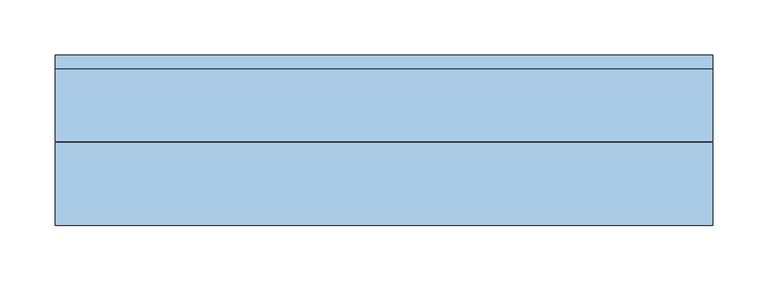
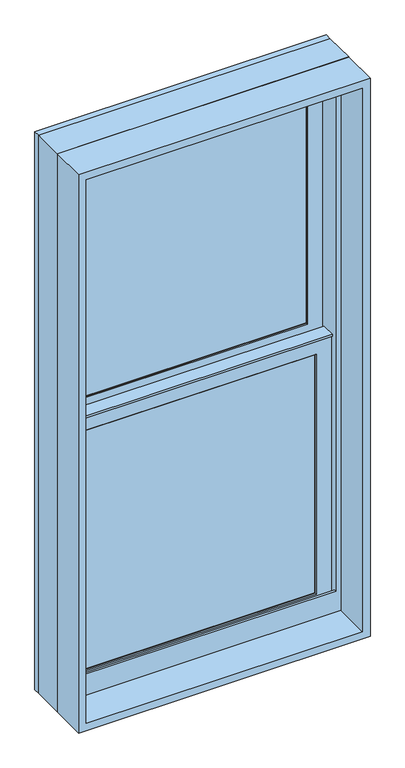
"""IFC4 building model written with IfcOpenShell, lengths in millimetres: window geometry, Window-Double_Hung-Marvin-Essential : ESDH2040."""

from ifc_helpers import new_model, si_unit, frame, origin, place, context, project, spatial, polyline, outline, extrude, faceted_brep, source, transform, mapped, element, save


def window_2436dc5c(model_context):
    return source(origin(), model_context, "Body", "SolidModel", [
        extrude(outline(polyline([(89.9583333, 20.6375), (89.9583333, 15.875), (70.9083333, 15.875), (70.9083333, 20.6375), (89.9583333, 20.6375)])), frame((0.0, 0.0, 1289.05), z_axis=(0.0, 0.0, 1.0), x_axis=(1.0, 0.0, 0.0)), (0.0, 0.0, 1.0), 527.05),
        extrude(outline(polyline([(-70.9083333, 20.6375), (-70.9083333, 15.875), (-89.9583333, 15.875), (-89.9583333, 20.6375), (-70.9083333, 20.6375)])), frame((0.0, 0.0, 1289.05), z_axis=(0.0, 0.0, 1.0), x_axis=(1.0, 0.0, 0.0)), (0.0, 0.0, 1.0), 527.05),
        extrude(outline(polyline([(241.3, 20.6375), (241.3, 15.875), (-241.3, 15.875), (-241.3, 20.6375), (241.3, 20.6375)])), frame((0.0, 0.0, 1543.05), z_axis=(0.0, 0.0, 1.0), x_axis=(1.0, 0.0, 0.0)), (0.0, 0.0, 1.0), 19.05),
        extrude(outline(polyline([(-89.9583333, 46.83125), (-89.9583333, 51.59375), (-70.9083333, 51.59375), (-70.9083333, 46.83125), (-89.9583333, 46.83125)])), frame((0.0, 0.0, 1854.2), z_axis=(0.0, 0.0, 1.0), x_axis=(1.0, 0.0, 0.0)), (0.0, 0.0, 1.0), 527.05),
        extrude(outline(polyline([(70.9083333, 46.83125), (70.9083333, 51.59375), (89.9583333, 51.59375), (89.9583333, 46.83125), (70.9083333, 46.83125)])), frame((0.0, 0.0, 1854.2), z_axis=(0.0, 0.0, 1.0), x_axis=(1.0, 0.0, 0.0)), (0.0, 0.0, 1.0), 527.05),
        extrude(outline(polyline([(-241.3, 46.83125), (-241.3, 51.59375), (241.3, 51.59375), (241.3, 46.83125), (-241.3, 46.83125)])), frame((0.0, 0.0, 2108.2), z_axis=(0.0, 0.0, 1.0), x_axis=(1.0, 0.0, 0.0)), (0.0, 0.0, 1.0), 19.05),
        extrude(outline(polyline([(89.9583333, 20.6375), (70.9083333, 20.6375), (70.9083333, 25.4), (89.9583333, 25.4), (89.9583333, 20.6375)])), frame((0.0, 0.0, 1289.05), z_axis=(0.0, 0.0, 1.0), x_axis=(1.0, 0.0, 0.0)), (0.0, 0.0, 1.0), 527.05),
        extrude(outline(polyline([(-70.9083333, 20.6375), (-89.9583333, 20.6375), (-89.9583333, 25.4), (-70.9083333, 25.4), (-70.9083333, 20.6375)])), frame((0.0, 0.0, 1289.05), z_axis=(0.0, 0.0, 1.0), x_axis=(1.0, 0.0, 0.0)), (0.0, 0.0, 1.0), 527.05),
        extrude(outline(polyline([(241.3, 20.6375), (-241.3, 20.6375), (-241.3, 25.4), (241.3, 25.4), (241.3, 20.6375)])), frame((0.0, 0.0, 1543.05), z_axis=(0.0, 0.0, 1.0), x_axis=(1.0, 0.0, 0.0)), (0.0, 0.0, 1.0), 19.05),
        extrude(outline(polyline([(-89.9583333, 56.35625), (-70.9083333, 56.35625), (-70.9083333, 51.59375), (-89.9583333, 51.59375), (-89.9583333, 56.35625)])), frame((0.0, 0.0, 1854.2), z_axis=(0.0, 0.0, 1.0), x_axis=(1.0, 0.0, 0.0)), (0.0, 0.0, 1.0), 527.05),
        extrude(outline(polyline([(70.9083333, 56.35625), (89.9583333, 56.35625), (89.9583333, 51.59375), (70.9083333, 51.59375), (70.9083333, 56.35625)])), frame((0.0, 0.0, 1854.2), z_axis=(0.0, 0.0, 1.0), x_axis=(1.0, 0.0, 0.0)), (0.0, 0.0, 1.0), 527.05),
        extrude(outline(polyline([(-241.3, 56.35625), (241.3, 56.35625), (241.3, 51.59375), (-241.3, 51.59375), (-241.3, 56.35625)])), frame((0.0, 0.0, 2108.2), z_axis=(0.0, 0.0, 1.0), x_axis=(1.0, 0.0, 0.0)), (0.0, 0.0, 1.0), 19.05),
        faceted_brep([(-268.2875, 5.6780605, 1846.1351748), (-268.2875, 5.6780605, 1841.5), (268.2875, 5.6780605, 1841.5), (268.2875, 5.6780605, 1846.1351748), (-268.2875, 34.8118605, 1846.1351748), (268.2875, 34.8118605, 1846.1351748), (268.2875, 34.8118605, 1841.5), (-268.2875, 34.8118605, 1841.5), (-268.2875, 30.1625, 1841.5), (-268.2875, 30.1625, 1262.0625), (-268.2875, 8.9241104, 1262.0625), (-268.2875, 8.9241104, 1841.5), (268.2875, 8.9241104, 1841.5), (268.2875, 30.1625, 1841.5), (268.2875, 8.9241104, 1262.0625), (268.2875, 30.1625, 1262.0625), (-252.4034752, 11.90625, 1827.2034752), (-252.4034752, 30.1625, 1827.2034752), (252.4034752, 30.1625, 1827.2034752), (252.4034752, 11.90625, 1827.2034752), (-235.74375, 10.4662439, 1810.54375), (-235.74375, 11.90625, 1810.54375), (235.74375, 11.90625, 1810.54375), (235.74375, 10.4662439, 1810.54375), (237.2858834, 8.9241104, 1812.0858834), (-237.2858834, 8.9241104, 1812.0858834), (252.4034752, 30.1625, 1277.9465248), (252.4034752, 11.90625, 1277.9465248), (235.74375, 11.90625, 1294.60625), (235.74375, 10.4662439, 1294.60625), (237.2858834, 8.9241104, 1293.0641166), (-252.4034752, 30.1625, 1277.9465248), (-252.4034752, 11.90625, 1277.9465248), (-235.74375, 11.90625, 1294.60625), (-235.74375, 10.4662439, 1294.60625), (-237.2858834, 8.9241104, 1293.0641166)], [[[0, 1, 2, 3]], [[4, 5, 6, 7]], [[1, 0, 4, 7, 8, 9, 10, 11]], [[2, 1, 11, 12]], [[7, 6, 13, 8]], [[3, 2, 12, 14, 15, 13, 6, 5]], [[0, 3, 5, 4]], [[16, 17, 18, 19]], [[20, 21, 22, 23]], [[20, 23, 24, 25]], [[19, 18, 26, 27]], [[23, 22, 28, 29]], [[24, 23, 29, 30]], [[27, 26, 31, 32]], [[29, 28, 33, 34]], [[30, 29, 34, 35]], [[15, 14, 10, 9]], [[15, 9, 8, 13], [18, 17, 31, 26]], [[17, 16, 32, 31]], [[16, 19, 27, 32], [22, 21, 33, 28]], [[21, 20, 34, 33]], [[20, 25, 35, 34]], [[10, 14, 12, 11], [25, 24, 30, 35]]]),
        extrude(outline(polyline([(38.5955581, 1827.2125), (33.5778968, 1827.2125), (33.5778968, 1828.8), (39.9405976, 1828.8), (39.9405976, 1827.2125), (61.515625, 1827.2125), (47.6307501, 1823.8975159), (38.5955581, 1823.8975159), (38.5955581, 1827.2125)])), frame((-268.2875, 0.0, 0.0), z_axis=(1.0, 0.0, 0.0), x_axis=(0.0, 1.0, 0.0)), (0.0, 0.0, 1.0), 536.575),
        faceted_brep([(298.45, 0.0, 1231.9), (298.45, 0.0, 2438.4), (-298.45, 0.0, 2438.4), (-298.45, 0.0, 1231.9), (272.25625, 0.0, 1293.01875), (-272.25625, 0.0, 1293.01875), (-272.25625, 0.0, 2412.20625), (272.25625, 0.0, 2412.20625), (272.25625, 3.96875, 1231.9), (-272.25625, 3.96875, 1231.9), (-272.25625, 3.96875, 1293.01875), (272.25625, 3.96875, 1293.01875), (-298.45, 65.6828125, 1231.9), (-272.25625, 65.6828125, 1231.9), (272.25625, 65.6828125, 1231.9), (298.45, 65.6828125, 1231.9), (-298.45, 65.6828125, 2438.4), (298.45, 65.6828125, 2438.4), (272.25625, 65.6828125, 2412.20625), (-272.25625, 65.6828125, 2412.20625)], [[[0, 1, 2, 3], [4, 5, 6, 7]], [[8, 9, 10, 11]], [[5, 4, 11, 10]], [[0, 3, 12, 13, 9, 8, 14, 15]], [[13, 12, 16, 17, 15, 14, 18, 19]], [[13, 19, 6, 5, 10, 9]], [[7, 6, 19, 18]], [[18, 14, 8, 11, 4, 7]], [[1, 0, 15, 17]], [[2, 1, 17, 16]], [[3, 2, 16, 12]]]),
        faceted_brep([(272.25625, 30.1625, 1835.15), (270.66875, 30.1625, 1835.15), (270.66875, 30.1625, 1256.2544613), (272.25625, 30.1625, 1256.2544613), (-270.66875, 30.1625, 1835.15), (-272.25625, 30.1625, 1835.15), (-272.25625, 30.1625, 1256.2544613), (-270.66875, 30.1625, 1256.2544613), (270.66875, 63.5, 1835.15), (272.25625, 63.5, 1835.15), (272.25625, 63.5, 1249.7743077), (270.66875, 63.5, 1249.7743077), (-272.25625, 63.5, 1835.15), (-270.66875, 63.5, 1835.15), (-270.66875, 63.5, 1249.7743077), (-272.25625, 63.5, 1249.7743077), (283.5108932, 3.96875, 1261.3460105), (283.5108932, 3.96875, 1231.9), (283.5108932, 65.6828125, 1231.9), (283.5108932, 65.6828125, 1249.350012), (-283.5108932, 3.96875, 1231.9), (-283.5108932, 3.96875, 1261.3460105), (-283.5108932, 65.6828125, 1249.350012), (-283.5108932, 65.6828125, 1231.9), (283.5108932, 78.58125, 1246.8428097), (-283.5108932, 78.58125, 1246.8428097), (-281.4971252, 68.2348864, 1248.8539391), (-263.53135, 68.2348864, 1248.8539391), (-263.53135, 65.6828125, 1249.350012), (263.53135, 65.6828125, 1249.350012), (263.53135, 68.2348864, 1248.8539391), (281.4971252, 68.2348864, 1248.8539391), (-298.45, 65.6828125, 1231.9), (-298.45, 78.5948249, 1231.9), (298.45, 78.5948249, 1231.9), (298.45, 65.6828125, 1231.9), (-298.45, 78.58125, 2438.4), (298.45, 78.58125, 2438.4), (283.5108932, 78.58125, 2423.4608932), (-283.5108932, 78.58125, 2423.4608932), (-298.45, 65.6828125, 2438.4), (-281.4971252, 68.2348864, 2421.4471252), (281.4971252, 68.2348864, 2421.4471252), (263.53135, 68.2348864, 2403.48135), (-263.53135, 68.2348864, 2403.48135), (-263.53135, 65.6828125, 2403.48135), (263.53135, 65.6828125, 2403.48135), (298.45, 65.6828125, 2438.4)], [[[0, 1, 2, 3]], [[4, 5, 6, 7]], [[8, 9, 10, 11]], [[12, 13, 14, 15]], [[1, 8, 11, 2]], [[9, 0, 3, 10]], [[1, 0, 9, 8]], [[5, 4, 13, 12]], [[5, 12, 15, 6]], [[13, 4, 7, 14]], [[16, 17, 18, 19]], [[20, 21, 22, 23]], [[24, 25, 26, 27, 28, 22, 21, 16, 19, 29, 30, 31], [3, 2, 11, 10], [7, 6, 15, 14]], [[17, 16, 21, 20]], [[17, 20, 23, 32, 33, 34, 35, 18]], [[34, 33, 36, 37], [25, 24, 38, 39]], [[33, 32, 40, 36]], [[39, 41, 26, 25]], [[41, 42, 31, 30, 43, 44, 27, 26]], [[44, 45, 28, 27]], [[40, 32, 23, 22, 28, 45, 46, 29, 19, 18, 35, 47]], [[36, 40, 47, 37]], [[39, 38, 42, 41]], [[44, 43, 46, 45]], [[34, 37, 47, 35]], [[42, 38, 24, 31]], [[46, 43, 30, 29]]]),
        extrude(outline(polyline([(248.44375, 11.90625), (-248.44375, 11.90625), (-248.44375, 15.08125), (248.44375, 15.08125), (248.44375, 11.90625)])), frame((0.0, 0.0, 1281.90625), z_axis=(0.0, 0.0, 1.0), x_axis=(1.0, 0.0, 0.0)), (0.0, 0.0, 1.0), 541.3375),
        extrude(outline(polyline([(248.44375, 42.8625), (-248.44375, 42.8625), (-248.44375, 46.0375), (248.44375, 46.0375), (248.44375, 42.8625)])), frame((0.0, 0.0, 1847.05625), z_axis=(0.0, 0.0, 1.0), x_axis=(1.0, 0.0, 0.0)), (0.0, 0.0, 1.0), 541.3375),
        faceted_brep([(-235.74375, 31.194477, 1810.54375), (-237.2858834, 32.7366104, 1812.0858834), (237.2858834, 32.7366104, 1812.0858834), (235.74375, 31.194477, 1810.54375), (-235.74375, 30.1625, 1810.54375), (235.74375, 30.1625, 1810.54375), (-268.2875, 32.7366104, 1843.0875), (-268.2875, 30.1625, 1843.0875), (268.2875, 30.1625, 1843.0875), (268.2875, 32.7366104, 1843.0875), (237.2858834, 32.7366104, 1293.0641166), (235.74375, 31.194477, 1294.60625), (235.74375, 30.1625, 1294.60625), (268.2875, 30.1625, 1262.0625), (268.2875, 32.7366104, 1262.0625), (-237.2858834, 32.7366104, 1293.0641166), (-235.74375, 31.194477, 1294.60625), (-235.74375, 30.1625, 1294.60625), (-268.2875, 30.1625, 1262.0625), (-268.2875, 32.7366104, 1262.0625)], [[[0, 1, 2, 3]], [[4, 0, 3, 5]], [[6, 7, 8, 9]], [[3, 2, 10, 11]], [[5, 3, 11, 12]], [[9, 8, 13, 14]], [[11, 10, 15, 16]], [[12, 11, 16, 17]], [[14, 13, 18, 19]], [[9, 14, 19, 6], [1, 15, 10, 2]], [[16, 15, 1, 0]], [[17, 16, 0, 4]], [[7, 18, 13, 8], [5, 12, 17, 4]], [[19, 18, 7, 6]]]),
        faceted_brep([(-252.4034752, 42.8625, 2392.3534752), (-252.4034752, 61.11875, 2392.3534752), (252.4034752, 61.11875, 2392.3534752), (252.4034752, 42.8625, 2392.3534752), (-235.74375, 41.4224939, 2375.69375), (-235.74375, 42.8625, 2375.69375), (235.74375, 42.8625, 2375.69375), (235.74375, 41.4224939, 2375.69375), (-237.2858834, 39.8803604, 2377.2358834), (237.2858834, 39.8803604, 2377.2358834), (-268.2875, 61.11875, 2408.2375), (-268.2875, 39.8803604, 2408.2375), (268.2875, 39.8803604, 2408.2375), (268.2875, 61.11875, 2408.2375), (252.4034752, 61.11875, 1843.0965248), (252.4034752, 42.8625, 1843.0965248), (235.74375, 42.8625, 1859.75625), (235.74375, 41.4224939, 1859.75625), (237.2858834, 39.8803604, 1858.2141166), (268.2875, 39.8803604, 1827.2125), (268.2875, 61.11875, 1827.2125), (-252.4034752, 61.11875, 1843.0965248), (-252.4034752, 42.8625, 1843.0965248), (-235.74375, 42.8625, 1859.75625), (-235.74375, 41.4224939, 1859.75625), (-237.2858834, 39.8803604, 1858.2141166), (-268.2875, 39.8803604, 1827.2125), (-268.2875, 61.11875, 1827.2125)], [[[0, 1, 2, 3]], [[4, 5, 6, 7]], [[8, 4, 7, 9]], [[10, 11, 12, 13]], [[3, 2, 14, 15]], [[7, 6, 16, 17]], [[9, 7, 17, 18]], [[13, 12, 19, 20]], [[15, 14, 21, 22]], [[17, 16, 23, 24]], [[18, 17, 24, 25]], [[20, 19, 26, 27]], [[13, 20, 27, 10], [1, 21, 14, 2]], [[22, 21, 1, 0]], [[3, 15, 22, 0], [5, 23, 16, 6]], [[24, 23, 5, 4]], [[25, 24, 4, 8]], [[11, 26, 19, 12], [9, 18, 25, 8]], [[27, 26, 11, 10]]]),
        faceted_brep([(-268.2875, 61.11875, 1827.2125), (-268.2875, 63.6928604, 1827.2125), (268.2875, 63.6928604, 1827.2125), (268.2875, 61.11875, 1827.2125), (-235.74375, 62.150727, 1859.75625), (-235.74375, 61.11875, 1859.75625), (235.74375, 61.11875, 1859.75625), (235.74375, 62.150727, 1859.75625), (-237.2858834, 63.6928604, 1858.2141166), (237.2858834, 63.6928604, 1858.2141166), (268.2875, 63.6928604, 2408.2375), (268.2875, 61.11875, 2408.2375), (235.74375, 61.11875, 2375.69375), (235.74375, 62.150727, 2375.69375), (237.2858834, 63.6928604, 2377.2358834), (-268.2875, 63.6928604, 2408.2375), (-268.2875, 61.11875, 2408.2375), (-235.74375, 61.11875, 2375.69375), (-235.74375, 62.150727, 2375.69375), (-237.2858834, 63.6928604, 2377.2358834)], [[[0, 1, 2, 3]], [[4, 5, 6, 7]], [[8, 4, 7, 9]], [[3, 2, 10, 11]], [[7, 6, 12, 13]], [[9, 7, 13, 14]], [[11, 10, 15, 16]], [[13, 12, 17, 18]], [[14, 13, 18, 19]], [[16, 15, 1, 0]], [[3, 11, 16, 0], [5, 17, 12, 6]], [[18, 17, 5, 4]], [[19, 18, 4, 8]], [[1, 15, 10, 2], [9, 14, 19, 8]]]),
        extrude(outline(polyline([(248.44375, 26.19375), (-248.44375, 26.19375), (-248.44375, 30.1625), (248.44375, 30.1625), (248.44375, 26.19375)])), frame((0.0, 0.0, 1281.90625), z_axis=(0.0, 0.0, 1.0), x_axis=(1.0, 0.0, 0.0)), (0.0, 0.0, 1.0), 541.3375),
        extrude(outline(polyline([(248.44375, 57.15), (-248.44375, 57.15), (-248.44375, 61.11875), (248.44375, 61.11875), (248.44375, 57.15)])), frame((0.0, 0.0, 1847.05625), z_axis=(0.0, 0.0, 1.0), x_axis=(1.0, 0.0, 0.0)), (0.0, 0.0, 1.0), 541.3375),
        extrude(outline(polyline([(2438.4, 298.45), (2438.4, -298.45), (1231.9, -298.45), (1231.9, 298.45), (2438.4, 298.45)]), holes=[polyline([(2422.525, 282.575), (1247.775, 282.575), (1247.775, -282.575), (2422.525, -282.575), (2422.525, 282.575)])]), frame((0.0, -76.2, 0.0), z_axis=(0.0, 1.0, 0.0), x_axis=(0.0, 0.0, 1.0)), (0.0, 0.0, 1.0), 75.40625),
    ])


if __name__ == "__main__":
    model = new_model("IFC4")
    model_context = context("Model", 3, world=origin())
    ifc_project = project(units=[si_unit("LENGTHUNIT", "METRE", prefix="MILLI")], contexts=[model_context])
    site = spatial("IfcSite", under=ifc_project)
    building = spatial("IfcBuilding", under=site)
    placement = place(None, origin())
    window_shape = window_2436dc5c(model_context)
    element("IfcWindow", 1, ObjectType="Window-Double_Hung-Marvin-Essential : ESDH2040", at=placement, inside=building, context=model_context, shape_type="MappedRepresentation", body=[
        mapped(window_shape, transform((0.0, 0.0, 0.0), x_axis=(1.0, 0.0, 0.0), y_axis=(0.0, 1.0, 0.0), z_axis=(0.0, 0.0, 1.0))),
    ])
    save(model, "model.ifc")

# Revit data of these elements
# Type "Window-Double_Hung-Marvin-Essential : ESDH2040"
#   Type Mark = "48"
#   Window Type = "Essential Double Hung"
#   Product data url = "https://bimobject.com/marvin-windows-and-doors/product/marvin-dhwau"
#   Product Guid = "c4a96547-874c-4385-91dc-a058adc19d98"
#   Frame = "All Ultrex"
#   Egress Window = "No"
#   URL = "www.marvin.com"
#   Model = "ESDH2040"
#   Manufacturer = "Marvin Windows and Doors"
#   Label Egress = ""
#   Glass Type = "IG Low E II with Argon"
#   Design Pressure = "DP50"
#   Description = "2448 DBHG"
#   Analytic Construction = "<None>"
#   Prairie Corner Width = 0' - 4"
#   Prairie Corner Height = 0' - 4"
#   Egress Width = 1' - 8 9/16"
#   Egress Height = 1' - 7 27/128"
#   Rough Width = 2' - 0"
#   Rough Height = 4' - 0"
#   Nominal Width = 2' - 0"
#   Nominal Height = 4' - 0"
#   Inset to Installation Flange [instance default] = 0' - 1"
#   Height = 3' - 11 1/2"
#   Egress Area = 2.74323 SF
#   Default Head Height = 8' - 0"
#   Width = 1' - 11 1/2"
#   Daylight Area = 5.23682 SF
#   DLO Width = 1' - 6 9/16"
#   DLO Height = 1' - 8 5/16"
#   Muntins Top Sash = yes
#   Lites Wide Top Sash = 3
#   Lites Wide Bottom Sash = 3
#   Lites High Top Sash = 2
#   Lites High Bottom Sash = 2
#   Lite Cut Prairie 9 = no
#   Lite Cut HV Grid = yes
#   Muntins Bottom Sash = yes
#   Label Visibility = no
#   Jamb Extension Visibility = yes
#   Edition number = 1
#   Interior Material = Ultrex-Marvin-Stonewhite
#   Glazing Material = Glass-Marvin-IG Low E II with Argon
#   Cladding Material = Ultrex-Marvin-Pebblegray
#   Wall Closure = (empty or 0)
#   Assembly Code = ""
# Element 1 (IfcWindow, "Window-Double_Hung-Marvin-Essential : ESDH2040")
#   Materials on its faces: "Ultrex-Marvin-Pebblegray", "Ultrex-Marvin-Stonewhite", "Glass-Marvin-IG Low E II with Argon"
# Materials
#   "Ultrex-Marvin-Stonewhite": class "Paint", colour RGB 250 251 245, transparency 0
#   "Glass-Marvin-IG Low E II with Argon": class "Glass", colour RGB 0 128 192, transparency 0.85
#   "Ultrex-Marvin-Pebblegray": class "Paint", colour RGB 189 185 173, transparency 0
